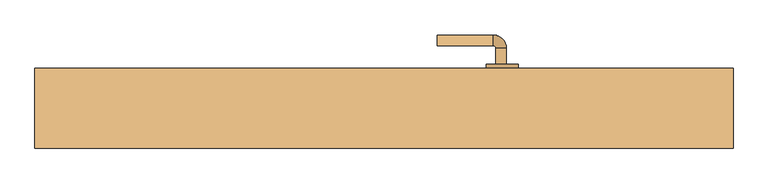
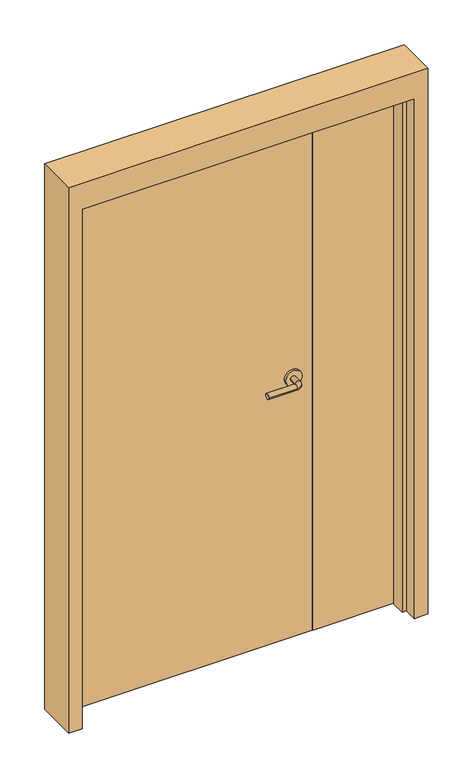
"""IFC4 building model written with IfcOpenShell, lengths in millimetres: door geometry, Дверь-Маятниковая-С полотнами разной ширины-Щитовая : 1310 x 2100 мм."""

from ifc_helpers import new_model, si_unit, point, frame, frame_2d, origin, origin_with_axes, place, context, project, spatial, polyline, circle_curve, ellipse_curve, trimmed, segment, composite_curve, outline, extrude, faceted_brep, source, transform, mapped, element, save
from ifc_brep_helpers import plane_surface, cylinder_surface, revolved_surface, advanced_brep


def door_47766967(model_context):
    return source(origin(), model_context, "Body", "SolidModel", [
        advanced_brep(
        [(229.59375, 15.85, 1000.0), (209.59375, 15.85, 1000.0), (229.59375, -14.15, 1000.0), (209.59375, -14.15, 1000.0), (204.59375, -19.15, 1000.0), (204.59375, -39.15, 1000.0), (99.59375, -39.15, 1000.0), (99.59375, -19.15, 1000.0)],
        [
            (0, 1, circle_curve(frame((219.59375, 15.85, 1000.0), z_axis=(0.0, 1.0, 0.0), x_axis=(-1.0, 0.0, 0.0)), 10.0)),
            (1, 0, circle_curve(frame((219.59375, 15.85, 1000.0), z_axis=(0.0, 1.0, 0.0), x_axis=(-1.0, 0.0, 0.0)), 10.0)),
            (0, 2),
            (2, 3, circle_curve(frame((219.59375, -14.15, 1000.0), z_axis=(0.0, 1.0, 0.0), x_axis=(-1.0, 0.0, 0.0)), 10.0)),
            (3, 1),
            (3, 2, circle_curve(frame((219.59375, -14.15, 1000.0), z_axis=(0.0, 1.0, 0.0), x_axis=(-1.0, 0.0, 0.0)), 10.0)),
            (4, 3, circle_curve(frame((204.59375, -14.15, 1000.0), z_axis=(0.0, 0.0, 1.0), x_axis=(1.0, 0.0, 0.0)), 5.0)),
            (2, 5, circle_curve(frame((204.59375, -14.15, 1000.0), z_axis=(0.0, 0.0, -1.0), x_axis=(1.0, 0.0, 0.0)), 25.0)),
            (5, 4, circle_curve(frame((204.59375, -29.15, 1000.0), z_axis=(1.0, 0.0, 0.0), x_axis=(0.0, 1.0, 0.0)), 10.0)),
            (4, 5, circle_curve(frame((204.59375, -29.15, 1000.0), z_axis=(1.0, 0.0, 0.0), x_axis=(0.0, 1.0, 0.0)), 10.0)),
            (6, 7, circle_curve(frame((99.59375, -29.15, 1000.0), z_axis=(-1.0, 0.0, 0.0), x_axis=(0.0, 1.0, 0.0)), 10.0)),
            (7, 6, circle_curve(frame((99.59375, -29.15, 1000.0), z_axis=(-1.0, 0.0, 0.0), x_axis=(0.0, 1.0, 0.0)), 10.0)),
            (5, 6),
            (7, 4),
        ],
        [
            plane_surface(frame((219.59375, 15.85, 1000.0), z_axis=(0.0, 1.0, 0.0), x_axis=(0.0, 0.0, 1.0))),
            cylinder_surface(frame((219.59375, 15.85, 1000.0), z_axis=(0.0, 1.0, 0.0), x_axis=(-1.0, 0.0, 0.0)), 10.0),
            revolved_surface(trimmed(ellipse_curve(frame((219.59375, -14.15, 1000.0), z_axis=(0.0, 1.0, 0.0), x_axis=(-1.0, 0.0, 0.0)), 10.0, 10.0), [point((229.59375, -14.15, 1000.0))], [point((209.59375, -14.15, 1000.0))], True, "CARTESIAN"), (204.59375, -14.15, 1000.0), (0.0, 0.0, -1.0)),
            revolved_surface(trimmed(ellipse_curve(frame((219.59375, -14.15, 1000.0), z_axis=(0.0, 1.0, 0.0), x_axis=(-1.0, 0.0, 0.0)), 10.0, 10.0), [point((209.59375, -14.15, 1000.0))], [point((229.59375, -14.15, 1000.0))], True, "CARTESIAN"), (204.59375, -14.15, 1000.0), (0.0, 0.0, -1.0)),
            plane_surface(frame((99.59375, -29.15, 1000.0), z_axis=(-1.0, 0.0, 0.0), x_axis=(0.0, 0.0, 1.0))),
            cylinder_surface(frame((204.59375, -29.15, 1000.0), z_axis=(1.0, 0.0, 0.0), x_axis=(0.0, 1.0, 0.0)), 10.0),
        ],
        [
            (0, [[1, 2]]),
            (1, [[-1, 3, 4, 5]]),
            (1, [[-2, -5, 6, -3]]),
            (2, [[7, -4, 8, 9]]),
            (3, [[-8, -6, -7, 10]]),
            (4, [[11, 12]]),
            (5, [[-9, 13, -12, 14]]),
            (5, [[-10, -14, -11, -13]]),
        ],
    ),
        extrude(outline(composite_curve([segment(trimmed(circle_curve(frame_2d((1000.0, 222.09375)), 30.0), [point((1000.0, 252.09375))], [point((1000.0, 192.09375))], False, "CARTESIAN"), True, "CONTINUOUS"), segment(trimmed(circle_curve(frame_2d((1000.0, 222.09375)), 30.0), [point((1000.0, 192.09375))], [point((1000.0, 252.09375))], False, "CARTESIAN"), True, "CONTINUOUS")], self_intersect=False)), frame((0.0, 15.85, 0.0), z_axis=(0.0, 1.0, 0.0), x_axis=(0.0, 0.0, 1.0)), (0.0, 0.0, 1.0), 8.0),
        advanced_brep(
        [(229.59375, 76.85, 1000.0), (209.59375, 76.85, 1000.0), (209.59375, 106.85, 1000.0), (229.59375, 106.85, 1000.0), (204.59375, 111.85, 1000.0), (204.59375, 131.85, 1000.0), (99.59375, 131.85, 1000.0), (99.59375, 111.85, 1000.0)],
        [
            (0, 1, circle_curve(frame((219.59375, 76.85, 1000.0), z_axis=(0.0, -1.0, 0.0), x_axis=(-1.0, 0.0, 0.0)), 10.0)),
            (1, 0, circle_curve(frame((219.59375, 76.85, 1000.0), z_axis=(0.0, -1.0, 0.0), x_axis=(-1.0, 0.0, 0.0)), 10.0)),
            (1, 2),
            (2, 3, circle_curve(frame((219.59375, 106.85, 1000.0), z_axis=(0.0, -1.0, 0.0), x_axis=(-1.0, 0.0, 0.0)), 10.0)),
            (3, 0),
            (3, 2, circle_curve(frame((219.59375, 106.85, 1000.0), z_axis=(0.0, -1.0, 0.0), x_axis=(-1.0, 0.0, 0.0)), 10.0)),
            (4, 5, circle_curve(frame((204.59375, 121.85, 1000.0), z_axis=(1.0, 0.0, 0.0), x_axis=(0.0, -1.0, 0.0)), 10.0)),
            (5, 3, circle_curve(frame((204.59375, 106.85, 1000.0), z_axis=(0.0, 0.0, -1.0), x_axis=(1.0, 0.0, 0.0)), 25.0)),
            (2, 4, circle_curve(frame((204.59375, 106.85, 1000.0), z_axis=(0.0, 0.0, 1.0), x_axis=(1.0, 0.0, 0.0)), 5.0)),
            (5, 4, circle_curve(frame((204.59375, 121.85, 1000.0), z_axis=(1.0, 0.0, 0.0), x_axis=(0.0, -1.0, 0.0)), 10.0)),
            (6, 7, circle_curve(frame((99.59375, 121.85, 1000.0), z_axis=(-1.0, 0.0, 0.0), x_axis=(0.0, -1.0, 0.0)), 10.0)),
            (7, 6, circle_curve(frame((99.59375, 121.85, 1000.0), z_axis=(-1.0, 0.0, 0.0), x_axis=(0.0, -1.0, 0.0)), 10.0)),
            (4, 7),
            (6, 5),
        ],
        [
            plane_surface(frame((219.59375, 76.85, 1000.0), z_axis=(0.0, -1.0, 0.0), x_axis=(0.0, 0.0, 1.0))),
            cylinder_surface(frame((219.59375, 76.85, 1000.0), z_axis=(0.0, -1.0, 0.0), x_axis=(-1.0, 0.0, 0.0)), 10.0),
            revolved_surface(trimmed(ellipse_curve(frame((219.59375, 106.85, 1000.0), z_axis=(0.0, 1.0, 0.0), x_axis=(-1.0, 0.0, 0.0)), 10.0, 10.0), [point((229.59375, 106.85, 1000.0))], [point((209.59375, 106.85, 1000.0))], True, "CARTESIAN"), (204.59375, 106.85, 1000.0), (0.0, 0.0, -1.0)),
            revolved_surface(trimmed(ellipse_curve(frame((219.59375, 106.85, 1000.0), z_axis=(0.0, 1.0, 0.0), x_axis=(-1.0, 0.0, 0.0)), 10.0, 10.0), [point((209.59375, 106.85, 1000.0))], [point((229.59375, 106.85, 1000.0))], True, "CARTESIAN"), (204.59375, 106.85, 1000.0), (0.0, 0.0, -1.0)),
            plane_surface(frame((99.59375, 121.85, 1000.0), z_axis=(-1.0, 0.0, 0.0), x_axis=(0.0, 0.0, 1.0))),
            cylinder_surface(frame((204.59375, 121.85, 1000.0), z_axis=(1.0, 0.0, 0.0), x_axis=(0.0, -1.0, 0.0)), 10.0),
        ],
        [
            (0, [[1, 2]]),
            (1, [[3, 4, 5, -2]]),
            (1, [[-5, 6, -3, -1]]),
            (2, [[7, 8, -4, 9]]),
            (3, [[10, -9, -6, -8]]),
            (4, [[11, 12]]),
            (5, [[13, -11, 14, -7]]),
            (5, [[-14, -12, -13, -10]]),
        ],
    ),
        extrude(outline(composite_curve([segment(trimmed(circle_curve(frame_2d((1000.0, 222.09375)), 30.0), [point((1000.0, 252.09375))], [point((1000.0, 192.09375))], False, "CARTESIAN"), True, "CONTINUOUS"), segment(trimmed(circle_curve(frame_2d((1000.0, 222.09375)), 30.0), [point((1000.0, 192.09375))], [point((1000.0, 252.09375))], False, "CARTESIAN"), True, "CONTINUOUS")], self_intersect=False)), frame((0.0, 68.85, 0.0), z_axis=(0.0, 1.0, 0.0), x_axis=(0.0, 0.0, 1.0)), (0.0, 0.0, 1.0), 8.0),
        extrude(outline(polyline([(605.0, 23.85), (296.6, 23.85), (296.6, 68.85), (605.0, 68.85), (605.0, 23.85)])), origin_with_axes(), (0.0, 0.0, 1.0), 2000.0),
        faceted_brep([(605.0, 19.0875, 0.0), (605.0, 68.85, 0.0), (655.0, 68.85, 0.0), (655.0, -81.15, 0.0), (605.0, -81.15, 0.0), (605.0, -31.9375, 0.0), (589.125, -31.9375, 0.0), (589.125, 19.0875, 0.0), (605.0, 19.0875, 2000.0), (605.0, 68.85, 2000.0), (-605.0, 68.85, 2000.0), (-605.0, 68.85, 0.0), (-655.0, 68.85, 0.0), (-655.0, 68.85, 2100.0), (655.0, 68.85, 2100.0), (655.0, -81.15, 2100.0), (-655.0, -81.15, 2100.0), (-655.0, -81.15, 0.0), (-605.0, -81.15, 0.0), (-605.0, -81.15, 2000.0), (605.0, -81.15, 2000.0), (605.0, -31.9375, 2000.0), (-605.0, -31.9375, 2000.0), (-605.0, -31.9375, 0.0), (-589.125, -31.9375, 0.0), (-589.125, -31.9375, 1984.125), (589.125, -31.9375, 1984.125), (589.125, 19.0875, 1984.125), (-589.125, 19.0875, 1984.125), (-589.125, 19.0875, 0.0), (-605.0, 19.0875, 0.0), (-605.0, 19.0875, 2000.0)], [[[0, 1, 2, 3, 4, 5, 6, 7]], [[1, 0, 8, 9]], [[2, 1, 9, 10, 11, 12, 13, 14]], [[3, 2, 14, 15]], [[4, 3, 15, 16, 17, 18, 19, 20]], [[5, 4, 20, 21]], [[6, 5, 21, 22, 23, 24, 25, 26]], [[7, 6, 26, 27]], [[0, 7, 27, 28, 29, 30, 31, 8]], [[9, 8, 31, 10]], [[20, 19, 22, 21]], [[26, 25, 28, 27]], [[12, 11, 30, 29, 24, 23, 18, 17]], [[11, 10, 31, 30]], [[13, 12, 17, 16]], [[19, 18, 23, 22]], [[25, 24, 29, 28]], [[15, 14, 13, 16]]]),
        extrude(outline(polyline([(293.4, 23.85), (-605.0, 23.85), (-605.0, 68.85), (293.4, 68.85), (293.4, 23.85)])), origin_with_axes(), (0.0, 0.0, 1.0), 2000.0),
    ])


if __name__ == "__main__":
    model = new_model("IFC4")
    model_context = context("Model", 3, world=origin())
    ifc_project = project(units=[si_unit("LENGTHUNIT", "METRE", prefix="MILLI")], contexts=[model_context])
    site = spatial("IfcSite", under=ifc_project)
    building = spatial("IfcBuilding", under=site)
    placement = place(None, origin())
    door_shape = door_47766967(model_context)
    element("IfcDoor", 1, ObjectType="Дверь-Маятниковая-С полотнами разной ширины-Щитовая : 1310 x 2100 мм", at=placement, inside=building, context=model_context, shape_type="MappedRepresentation", body=[
        mapped(door_shape, transform((0.0, 0.0, 0.0), x_axis=(1.0, 0.0, 0.0), y_axis=(0.0, 1.0, 0.0), z_axis=(0.0, 0.0, 1.0))),
    ])
    save(model, "model.ifc")

# Revit data of these elements
# Type "Дверь-Маятниковая-С полотнами разной ширины-Щитовая : 1310 x 2100 мм"
#   Type Mark = "150"
#   Assembly Code = "C1020300"
#   Analytic Construction = "Деревянный"
#   Ширина большой панели = 900 mm
#   W = 310 mm
#   Thickness = 45 mm
#   Thermal Resistance (R) = 0.455703 (m²·K)/W
#   Угол поворота [instance default] = 90°
#   Высота планки = 1000 mm
#   Rough Width [instance default] = 1310 mm
#   Rough Height [instance default] = 2100 mm
#   Высота проема в кирпичном каркасе [instance default] = 100 mm
#   Ширина проема в кирпичном каркасе [instance default] = 100 mm
#   Расчет вставки [instance default] = 105 mm
#   Кирпичная вставка [instance default] = 25 mm
#   Height = 2000 mm
#   Width = 1210 mm
#   Heat Transfer Coefficient (U) = 2.19465 W/(m²·K)
#   Глубина кирпичного каркаса = 150 mm
#   Кирпичный каркас [instance default] = yes
#   Каркас стены сухой кладки [instance default] = no
#   Материал панели = Древесина - Береза
#   Материал каркаса = Металл - Окрашенный - Серый 2
#   Материал дверной ручки = Алюминий
#   Visual Light Transmittance = 0
#   Solar Heat Gain Coefficient = 0
#   Wall Closure = (empty or 0)
#   Function = (empty or 0)
# Element 1 (IfcDoor, "Дверь-Маятниковая-С полотнами разной ширины-Щитовая : 1310 x 2100 мм")
#   Расчет вставки = 80 mm
#   Кирпичная вставка = 0 mm
#   Materials on its faces: "Алюминий", "Металл - Окрашенный - Серый 2", "Древесина - Береза"
# Materials
#   "Древесина - Береза": class "Древесина", colour RGB 166 116 52, transparency 0, Cost = 0
#   "Металл - Окрашенный - Серый 2": class "Краска", colour RGB 104 104 104, transparency 0, Cost = 0
#   "Алюминий": class "Металл", colour RGB 247 247 247, transparency 0
